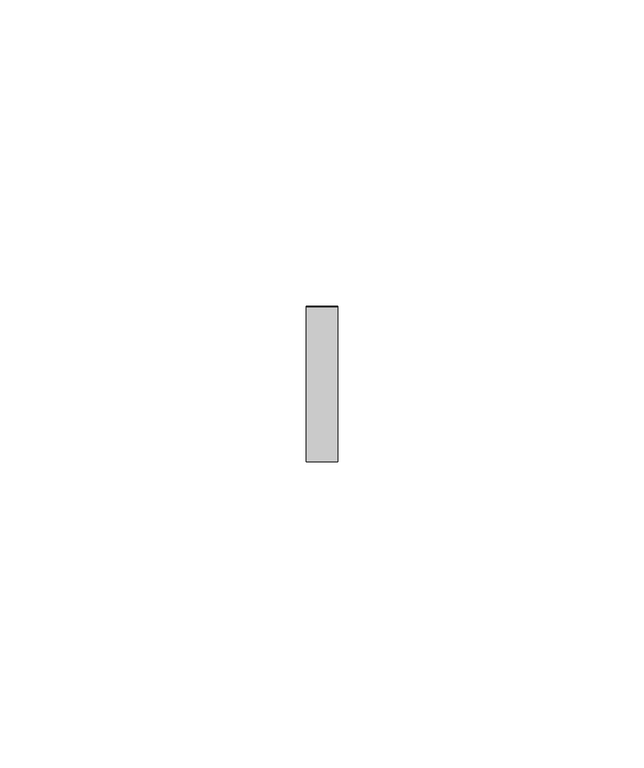
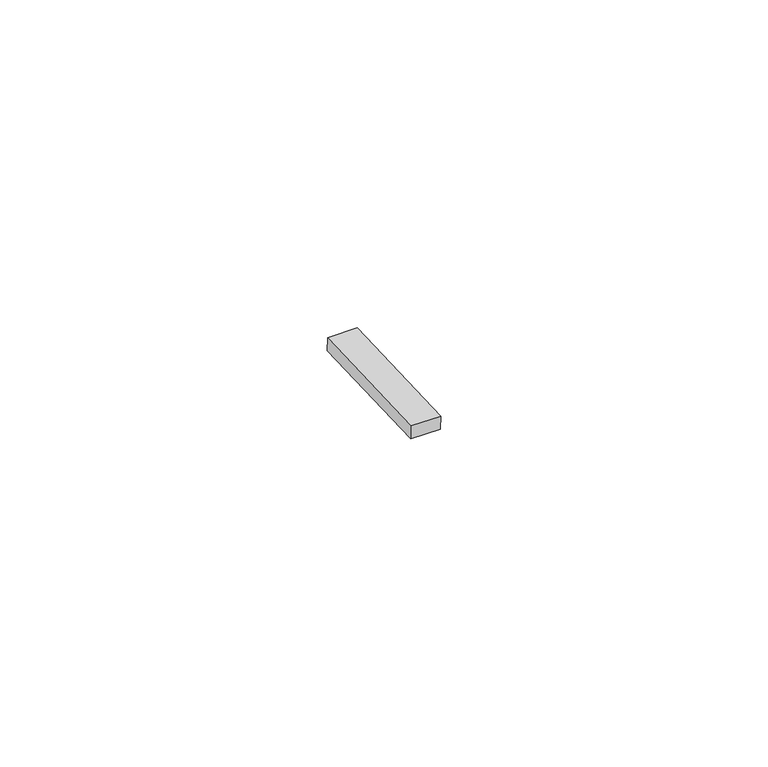
"""IFC4 building model written with IfcOpenShell, lengths in millimetres: proxy geometry, Inner panel:Inner panel:1:Inner panel:1 : Inner panel:Inner panel:300324:2:Inner panel:1:Inner panel:1 : Inner panel:Inner panel:300324:2 : Inner panel:Inner panel:1:Inner panel:1 : Inner panel:Inner panel:300324:300043:114 : Inner panel:Inner panel:1:Inner panel:1 : Inner panel:Inner panel:300324:2:Inner panel:1:Inner panel:1 : Inner panel:Inner panel:300324:2 : Inner panel:Inner panel:1:Inner panel:1 : Inner panel:Inner panel:300324:300043:308120."""

from ifc_helpers import new_model, si_unit, frame, origin, place, context, project, spatial, polyline, outline, extrude, source, transform, mapped, element, save


def generic_models_42414af7(model_context):
    return source(origin(), model_context, "Body", "SweptSolid", [
        extrude(outline(polyline([(0.0, -25.3999999), (0.0, 0.0), (5.2138089, 0.0), (5.2138089, -25.3999999), (0.0, -25.3999999)])), frame((593936.595117, -577413.7950993, 4016.01903), z_axis=(0.0, -0.041630544712223896, 0.9991330730923502), x_axis=(-1.0, 0.0, 0.0)), (0.0, 0.0, 1.0), 2.4763745),
    ])


if __name__ == "__main__":
    model = new_model("IFC4")
    model_context = context("Model", 3, world=origin())
    ifc_project = project(units=[si_unit("LENGTHUNIT", "METRE", prefix="MILLI")], contexts=[model_context])
    site = spatial("IfcSite", under=ifc_project)
    building = spatial("IfcBuilding", under=site)
    placement = place(None, origin())
    generic_models_shape = generic_models_42414af7(model_context)
    element("IfcBuildingElementProxy", 1, Name="Inner panel:Inner panel:1:Inner panel:1 : Inner panel:Inner panel:300324:2:Inner panel:1:Inner panel:1 : Inner panel:Inner panel:300324:2 : Inner panel:Inner panel:1:Inner panel:1 : Inner panel:Inner panel:300324:300043:114 : Inner panel:Inner panel:1:Inner panel:1 : Inner panel:Inner panel:300324:2:Inner panel:1:Inner panel:1 : Inner panel:Inner panel:300324:2 : Inner panel:Inner panel:1:Inner panel:1 : Inner panel:Inner panel:300324:300043:308120", ObjectType="Inner panel:Inner panel:1:Inner panel:1 : Inner panel:Inner panel:300324:2:Inner panel:1:Inner panel:1 : Inner panel:Inner panel:300324:2 : Inner panel:Inner panel:1:Inner panel:1 : Inner panel:Inner panel:300324:300043:114 : Inner panel:Inner panel:1:Inner panel:1 : Inner panel:Inner panel:300324:2:Inner panel:1:Inner panel:1 : Inner panel:Inner panel:300324:2 : Inner panel:Inner panel:1:Inner panel:1 : Inner panel:Inner panel:300324:300043:308120", at=placement, inside=building, context=model_context, shape_type="MappedRepresentation", body=[
        mapped(generic_models_shape, transform((0.0, 0.0, 0.0), x_axis=(1.0, 0.0, 0.0), y_axis=(0.0, 1.0, 0.0), z_axis=(0.0, 0.0, 1.0))),
    ])
    save(model, "model.ifc")

# Revit data of these elements
# Type "Inner panel:Inner panel:1:Inner panel:1 : Inner panel:Inner panel:300324:2:Inner panel:1:Inner panel:1 : Inner panel:Inner panel:300324:2 : Inner panel:Inner panel:1:Inner panel:1 : Inner panel:Inner panel:300324:300043:114 : Inner panel:Inner panel:1:Inner panel:1 : Inner panel:Inner panel:300324:2:Inner panel:1:Inner panel:1 : Inner panel:Inner panel:300324:2 : Inner panel:Inner panel:1:Inner panel:1 : Inner panel:Inner panel:300324:300043:308120"
#   NameOverride = "Inner panel:Inner panel:1:Inner panel:1 : Inner panel:Inner panel:300324:2:Inner panel:1:Inner panel:1 : Inner panel:Inner panel:300324:2 : Inner panel:Inner panel:1:Inner panel:1 : Inner panel:Inner panel:300324:300043:308120"
#   ObjectTypeOverride = "Inner panel:1:Inner panel:1 : Inner panel:Inner panel:300324:2 : Inner panel:Inner panel:1:Inner panel:1 : Inner panel:Inner panel:300324:300043"
#   Reference = "Inner panel"
#   Tag = "308120"
# Element 1 (IfcBuildingElementProxy, "Inner panel:Inner panel:1:Inner panel:1 : Inner panel:Inner panel:300324:2:Inner panel:1:Inner panel:1 : Inner panel:Inner panel:300324:2 : Inner panel:Inner panel:1:Inner panel:1 : Inner panel:Inner panel:300324:300043:114 : Inner panel:Inner panel:1:Inner panel:1 : Inner panel:Inner panel:300324:2:Inner panel:1:Inner panel:1 : Inner panel:Inner panel:300324:2 : Inner panel:Inner panel:1:Inner panel:1 : Inner panel:Inner panel:300324:300043:308120")
#   Materials on its faces: "AT CLIP - 1\" WIDE NON ABSORBENT, WEATHER-RESISTANT NEOPRENE/EPDM/SBR FOAM"
# Materials
#   "AT CLIP - 1\" WIDE NON ABSORBENT, WEATHER-RESISTANT NEOPRENE/EPDM/SBR FOAM": class "Generic", colour RGB 85 85 85, transparency 0, Cost = 0
